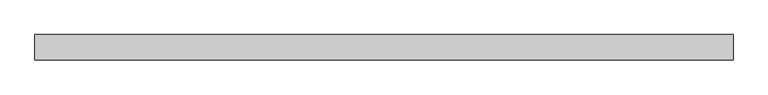
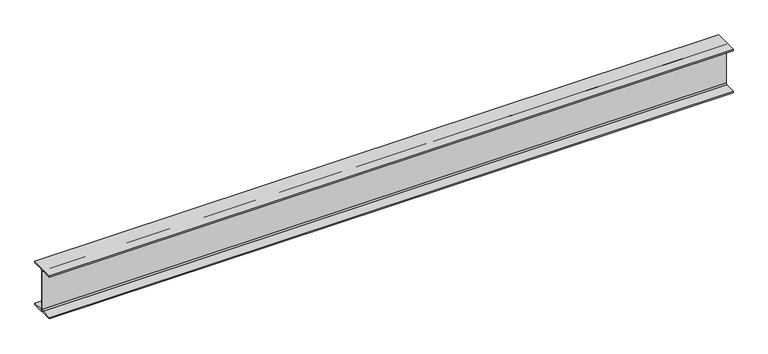
"""IFC4 building model written with IfcOpenShell, lengths in millimetres: beam geometry, Steel Beam_H-KSD3502 : H_SB_ASB_H-250x125x6x9."""

from ifc_helpers import new_model, si_unit, point, frame, frame_2d, origin, place, context, project, spatial, polyline, circle_curve, trimmed, segment, composite_curve, outline, extrude, source, transform, mapped, element, save


def beam_873fa0fc(model_context):
    return source(origin(), model_context, "Body", "SweptSolid", [
        extrude(outline(composite_curve([segment(polyline([(82.5, -141.5), (82.5, -151.7), (-82.5, -151.7), (-82.5, -141.5), (-11.9, -141.5)]), True, "CONTINUOUS"), segment(trimmed(circle_curve(frame_2d((-11.9, -132.6)), 8.9), [point((-11.9, -141.5))], [point((-3.0, -132.6))], True, "CARTESIAN"), True, "CONTINUOUS"), segment(polyline([(-3.0, -132.6), (-3.0, 132.6)]), True, "CONTINUOUS"), segment(trimmed(circle_curve(frame_2d((-11.9, 132.6)), 8.9), [point((-3.0, 132.6))], [point((-11.9, 141.5))], True, "CARTESIAN"), True, "CONTINUOUS"), segment(polyline([(-11.9, 141.5), (-82.5, 141.5), (-82.5, 151.7), (82.5, 151.7), (82.5, 141.5), (11.9, 141.5)]), True, "CONTINUOUS"), segment(trimmed(circle_curve(frame_2d((11.9, 132.6)), 8.9), [point((11.9, 141.5))], [point((3.0, 132.6))], True, "CARTESIAN"), True, "CONTINUOUS"), segment(polyline([(3.0, 132.6), (3.0, -132.6)]), True, "CONTINUOUS"), segment(trimmed(circle_curve(frame_2d((11.9, -132.6)), 8.9), [point((3.0, -132.6))], [point((11.9, -141.5))], True, "CARTESIAN"), True, "CONTINUOUS"), segment(polyline([(11.9, -141.5), (82.5, -141.5)]), True, "CONTINUOUS")], self_intersect=False)), frame((-2164.4729123, 0.0, 0.0), z_axis=(1.0, 0.0, 0.0), x_axis=(0.0, 1.0, 0.0)), (0.0, 0.0, 1.0), 4526.7729123),
    ])


if __name__ == "__main__":
    model = new_model("IFC4")
    model_context = context("Model", 3, world=origin())
    ifc_project = project(units=[si_unit("LENGTHUNIT", "METRE", prefix="MILLI")], contexts=[model_context])
    site = spatial("IfcSite", under=ifc_project)
    building = spatial("IfcBuilding", under=site)
    placement = place(None, origin())
    beam_shape = beam_873fa0fc(model_context)
    element("IfcBeam", 1, ObjectType="Steel Beam_H-KSD3502 : H_SB_ASB_H-250x125x6x9", at=placement, inside=building, context=model_context, shape_type="MappedRepresentation", body=[
        mapped(beam_shape, transform((0.0, 0.0, 0.0), x_axis=(1.0, 0.0, 0.0), y_axis=(0.0, 1.0, 0.0), z_axis=(0.0, 0.0, 1.0))),
    ])
    save(model, "model.ifc")

# Revit data of these elements
# Type "Steel Beam_H-KSD3502 : H_SB_ASB_H-250x125x6x9"
#   Width = 12.5 cm
#   Web Thickness = 0.6 cm
#   Web Fillet = 1.2 cm
#   Warping Constant = 42539.8 cm⁶
#   Torsional Moment of Inertia = 7.8102 cm⁴
#   Torsional Modulus = 1.0 cm³
#   Section Area = 37.66 cm²
#   Plastic Modulus weak axis = 73.1 cm³
#   Plastic Modulus strong axis = 366.0 cm³
#   Perimeter = 0.97 m²/m
#   Nominal Weight = 29.60 kgf/m
#   Moment of Inertia weak axis = 294.00 cm⁴
#   Moment of Inertia strong axis = 4050.00 cm⁴
#   Height = 25.0 cm
#   Flange Thickness = 0.9 cm
#   Elastic Modulus weak axis = 47.0 cm³
#   Elastic Modulus strong axis = 324.0 cm³
#   Centroid Vertical = 12.5 cm
#   Centroid Horizontal = 6.25 cm
#   Length [instance default] = 1.5240 m
#   Structural Material [instance default] = Steel, 45-345
#   Assembly Code = ""
# Element 1 (IfcBeam, "Steel Beam_H-KSD3502 : H_SB_ASB_H-250x125x6x9")
#   Structural Material = none
# Materials
#   "Steel, 45-345": class "Metal", colour RGB 189 187 185, transparency 0, Description = "Steel 345 MPa", Cost = 0
